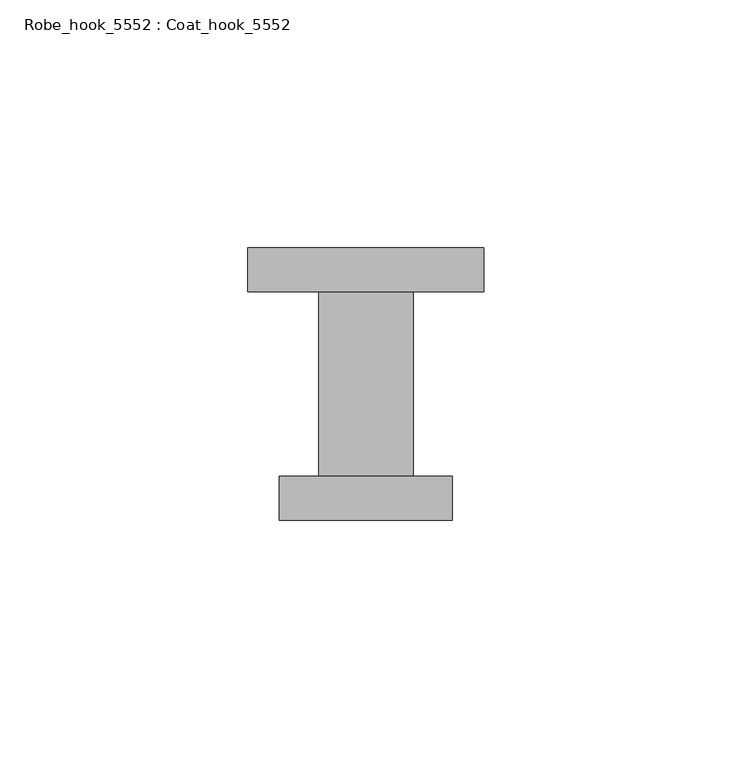
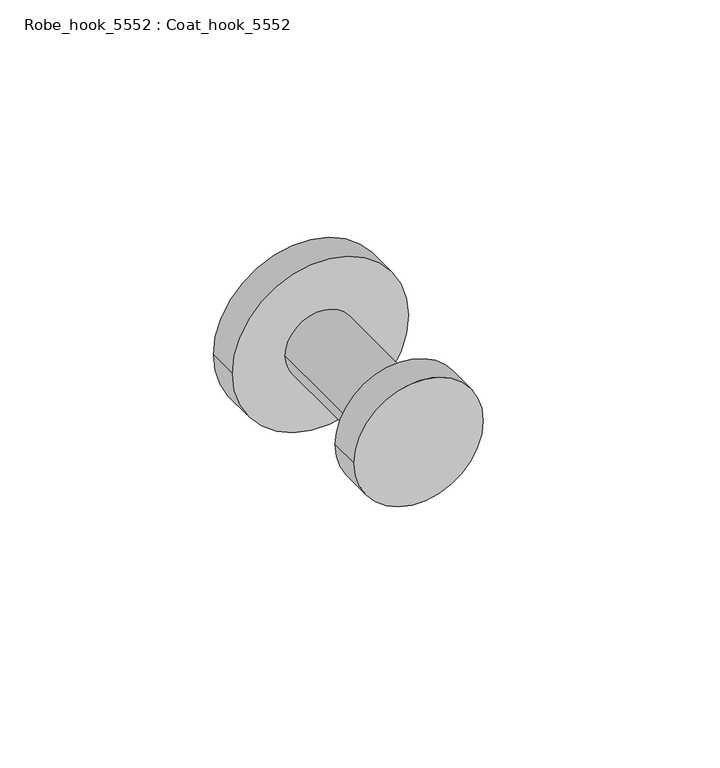
"""IFC4 building model written with IfcOpenShell, lengths in millimetres: proxy geometry, Robe_hook_5552 : Coat_hook_5552."""

from ifc_helpers import new_model, si_unit, point, frame, frame_2d, origin, place, context, project, spatial, circle_curve, trimmed, segment, composite_curve, outline, extrude, source, transform, mapped, element, save


def robe_hook_5552_coat_hook_5552_aa4161fa(model_context):
    return source(origin(), model_context, "Body", "SweptSolid", [
        extrude(outline(composite_curve([segment(trimmed(circle_curve(frame_2d((1371.6, 0.0)), 17.4626016), [point((1371.6, 17.4626016))], [point((1371.6, -17.4626016))], False, "CARTESIAN"), True, "CONTINUOUS"), segment(trimmed(circle_curve(frame_2d((1371.6, 0.0)), 17.4626016), [point((1371.6, -17.4626016))], [point((1371.6, 17.4626016))], False, "CARTESIAN"), True, "CONTINUOUS")], self_intersect=False)), frame((0.0, -54.9422932, 0.0), z_axis=(0.0, 1.0, 0.0), x_axis=(0.0, 0.0, 1.0)), (0.0, 0.0, 1.0), 8.9023917),
        extrude(outline(composite_curve([segment(trimmed(circle_curve(frame_2d((1371.6, 0.0)), 9.525), [point((1371.6, 9.525))], [point((1371.6, -9.525))], False, "CARTESIAN"), True, "CONTINUOUS"), segment(trimmed(circle_curve(frame_2d((1371.6, 0.0)), 9.525), [point((1371.6, -9.525))], [point((1371.6, 9.525))], False, "CARTESIAN"), True, "CONTINUOUS")], self_intersect=False)), frame((0.0, -46.0399015, 0.0), z_axis=(0.0, 1.0, 0.0), x_axis=(0.0, 0.0, 1.0)), (0.0, 0.0, 1.0), 37.1375098),
        extrude(outline(composite_curve([segment(trimmed(circle_curve(frame_2d((1371.6, 0.0)), 23.8125), [point((1371.6, 23.8125))], [point((1371.6, -23.8125))], False, "CARTESIAN"), True, "CONTINUOUS"), segment(trimmed(circle_curve(frame_2d((1371.6, 0.0)), 23.8125), [point((1371.6, -23.8125))], [point((1371.6, 23.8125))], False, "CARTESIAN"), True, "CONTINUOUS")], self_intersect=False)), frame((0.0, -8.9023917, 0.0), z_axis=(0.0, 1.0, 0.0), x_axis=(0.0, 0.0, 1.0)), (0.0, 0.0, 1.0), 8.9023917),
    ])


if __name__ == "__main__":
    model = new_model("IFC4")
    model_context = context("Model", 3, world=origin())
    ifc_project = project(units=[si_unit("LENGTHUNIT", "METRE", prefix="MILLI")], contexts=[model_context])
    site = spatial("IfcSite", under=ifc_project)
    building = spatial("IfcBuilding", under=site)
    placement = place(None, origin())
    robe_hook_5552_coat_hook_5552_shape = robe_hook_5552_coat_hook_5552_aa4161fa(model_context)
    element("IfcBuildingElementProxy", 1, Name="Robe_hook_5552 : Coat_hook_5552", ObjectType="Robe_hook_5552 : Coat_hook_5552", at=placement, inside=building, context=model_context, shape_type="MappedRepresentation", body=[
        mapped(robe_hook_5552_coat_hook_5552_shape, transform((0.0, 0.0, 0.0), x_axis=(1.0, 0.0, 0.0), y_axis=(0.0, 1.0, 0.0), z_axis=(0.0, 0.0, 1.0))),
    ])
    save(model, "model.ifc")

# Revit data of these elements
# Type "Robe_hook_5552 : Coat_hook_5552"
#   Keynote = "M10281600.03"
